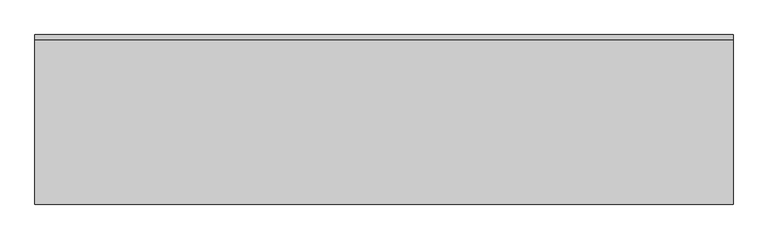
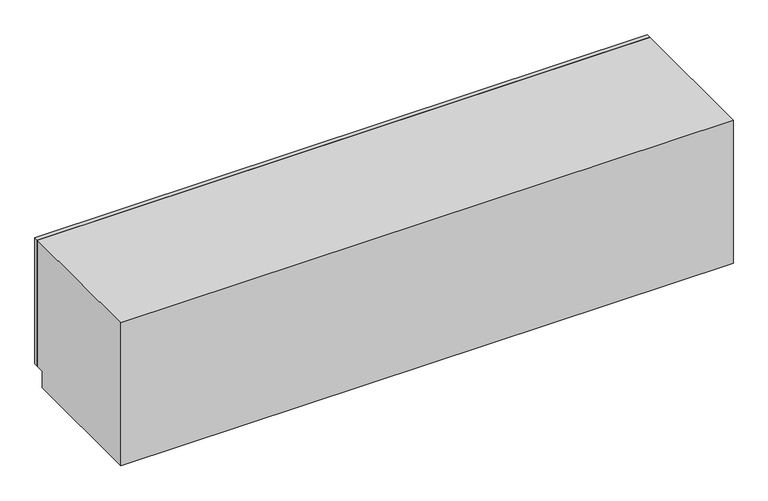
"""IFC4 building model written with IfcOpenShell, lengths in millimetres: furniture geometry, OD_CW_Base Cabinet : OD_CW_Base Cabinet."""

from ifc_helpers import new_model, si_unit, frame, origin, place, context, project, spatial, polyline, outline, extrude, source, transform, mapped, element, save


def furniture_b94af5d3(model_context):
    return source(origin(), model_context, "Body", "SweptSolid", [
        extrude(outline(polyline([(18.7377049, 228.6), (18.7377049, 254.0), (3573.4373466, 254.0), (3573.4373466, 228.6), (18.7377049, 228.6)])), frame((0.0, 0.0, 101.6), z_axis=(0.0, 0.0, 1.0), x_axis=(1.0, 0.0, 0.0)), (0.0, 0.0, 1.0), 774.7),
        extrude(outline(polyline([(228.6, 876.3), (228.6, 101.6), (177.8, 101.6), (177.8, 0.0), (-609.6, 0.0), (-609.6, 876.3), (228.6, 876.3)])), frame((18.7377049, 0.0, 0.0), z_axis=(1.0, 0.0, 0.0), x_axis=(0.0, 1.0, 0.0)), (0.0, 0.0, 1.0), 3554.6996417),
    ])


if __name__ == "__main__":
    model = new_model("IFC4")
    model_context = context("Model", 3, world=origin())
    ifc_project = project(units=[si_unit("LENGTHUNIT", "METRE", prefix="MILLI")], contexts=[model_context])
    site = spatial("IfcSite", under=ifc_project)
    building = spatial("IfcBuilding", under=site)
    placement = place(None, origin())
    furniture_shape = furniture_b94af5d3(model_context)
    element("IfcFurniture", 1, ObjectType="OD_CW_Base Cabinet : OD_CW_Base Cabinet", at=placement, inside=building, context=model_context, shape_type="MappedRepresentation", body=[
        mapped(furniture_shape, transform((0.0, 0.0, 0.0), x_axis=(1.0, 0.0, 0.0), y_axis=(0.0, 1.0, 0.0), z_axis=(0.0, 0.0, 1.0))),
    ])
    save(model, "model.ifc")

# Revit data of these elements
# Type "OD_CW_Base Cabinet : OD_CW_Base Cabinet"
#   OD_CW_Width [instance default] = 2' - 10"
#   OD_CW_Length [instance default] = 8' - 0"
#   OD_CW_Height [instance default] = 2' - 3"
#   Depth = 2' - 0"
#   Height = 3' - 0"
#   Width = 4' - 0"
#   OD_CW_Material_Front Panel [instance default] = none
#   OD_CW_Material_Body [instance default] = none
# Element 1 (IfcFurniture, "OD_CW_Base Cabinet : OD_CW_Base Cabinet")
#   OD_CW_Length = 11' - 7.9488"
#   OD_CW_Height = 2' - 10 1/2"
#   OD_CW_Material_Front Panel = WOOD-OAKFIRE
#   OD_CW_Material_Body = WOOD-OAKFIRE
#   Materials on its faces: "WOOD-OAKFIRE"
# Materials
#   "WOOD-OAKFIRE": class "Wood", colour RGB 198 202 183, transparency 0, Description = "Generic wood", Cost = 0
